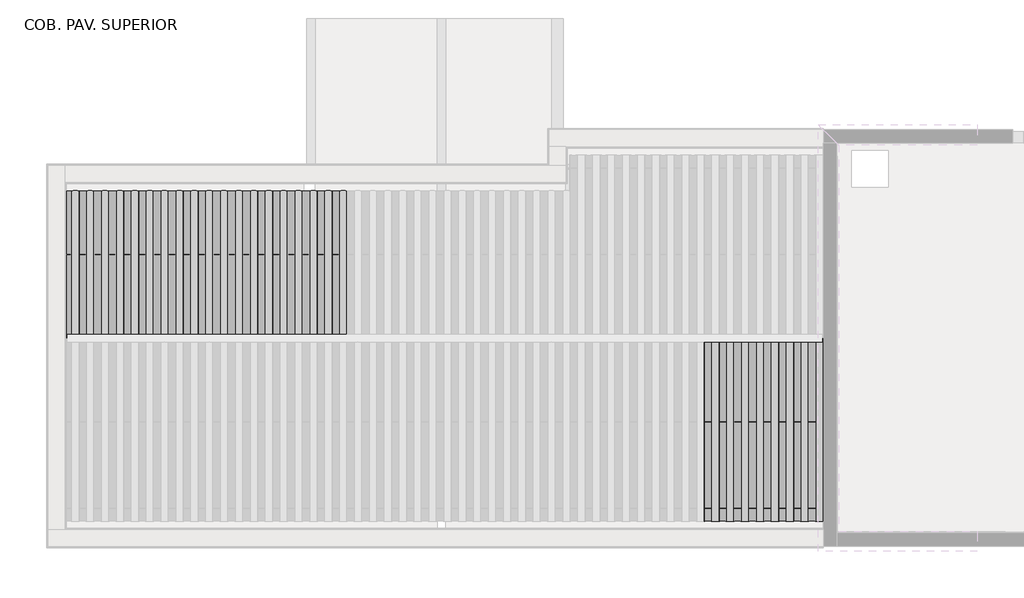
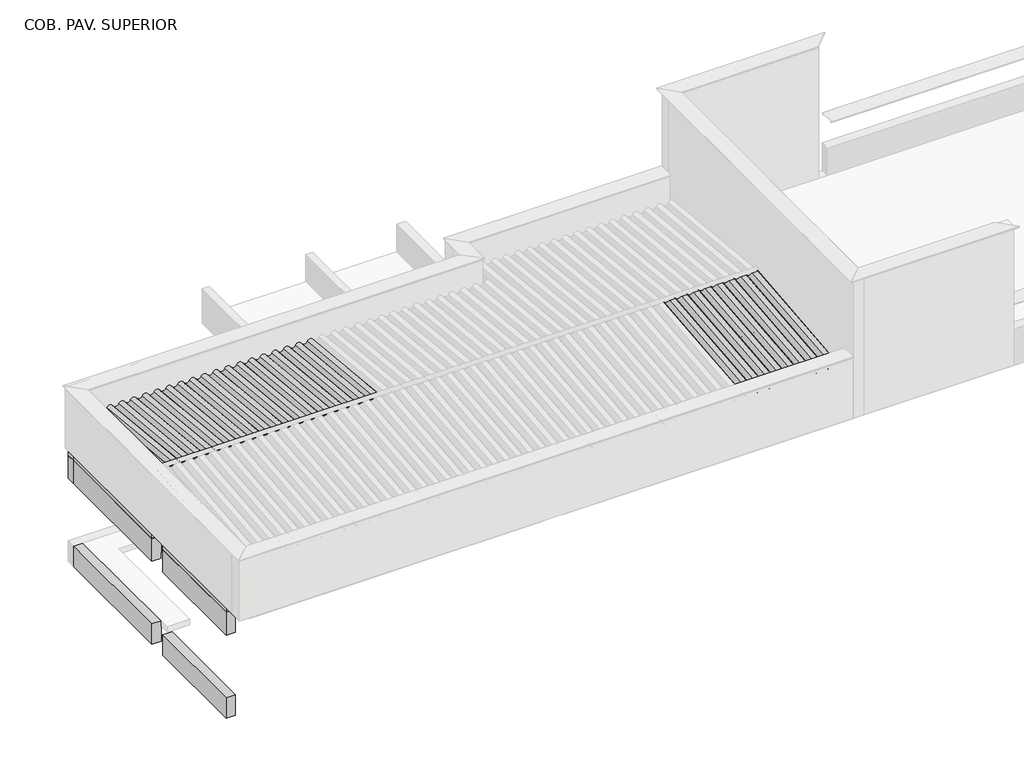
# One storey, part 3 of 7: 39 beams, 5 columns.
"""IFC4 building model written with IfcOpenShell, lengths in millimetres."""

import ifcopenshell
import ifcopenshell.guid

model = None  # the IFC model being written
_history = None  # IfcOwnerHistory: only IFC2X3 demands one
_inside = {}  # id of a spatial element -> (the spatial element, [elements in it])
_under = {}  # id of a project, library or spatial element -> (it, [spatial elements below it])
_declared = {}  # id of a project -> (the project, [libraries it declares])
_typed = {}  # id of a type object -> (the type object, [elements of that type])
_made_of = {}  # id of a material, layer set ... -> (it, [elements and type objects made of it])


def new_model(schema):
    """Start an empty IFC model of exactly this schema.

    Asked for "IFC4X3", IfcOpenShell would pick the latest addendum, in which some entities
    have other attributes; the version numbers below select the first issue.
    IFC2X3 requires an IfcOwnerHistory on every rooted entity: one is made here for all.
    """
    global model, _history
    if schema == "IFC4X3":
        model = ifcopenshell.file(schema_version=(4, 3, 0, 0))
    else:
        model = ifcopenshell.file(schema=schema)
    _inside.clear()
    _under.clear()
    _declared.clear()
    _typed.clear()
    _made_of.clear()
    _history = None
    if model.schema == "IFC2X3":
        org = make("IfcOrganization", Name="unknown")
        user = make(
            "IfcPersonAndOrganization",
            ThePerson=make("IfcPerson", FamilyName="unknown"),
            TheOrganization=org,
        )
        app = make(
            "IfcApplication",
            ApplicationDeveloper=org,
            Version="unknown",
            ApplicationFullName="unknown",
            ApplicationIdentifier="unknown",
        )
        _history = make(
            "IfcOwnerHistory",
            OwningUser=user,
            OwningApplication=app,
            ChangeAction="ADDED",
            CreationDate=0,
        )
    return model


def make(cls, **values):
    """One entity of the class cls with the attributes given. An attribute that is None is left unset."""
    return model.create_entity(
        cls, **{name: value for name, value in values.items() if value is not None}
    )


def rooted(cls, **values):
    """An entity with a GlobalId (a new one), such as an element, a storey or a relation."""
    return make(cls, GlobalId=ifcopenshell.guid.new(), OwnerHistory=_history, **values)


def si_unit(unit_type, name, prefix=None):
    """IfcSIUnit, for example si_unit("LENGTHUNIT", "METRE", prefix="MILLI")."""
    return make("IfcSIUnit", UnitType=unit_type, Prefix=prefix, Name=name)


def assignment(units):
    """IfcUnitAssignment: the units of a project."""
    return None if units is None else make("IfcUnitAssignment", Units=units)


def point(xyz):
    """IfcCartesianPoint."""
    return None if xyz is None else make("IfcCartesianPoint", Coordinates=xyz)


def direction(xyz):
    """IfcDirection."""
    return None if xyz is None else make("IfcDirection", DirectionRatios=xyz)


def frame(location, z_axis=None, x_axis=None):
    """IfcAxis2Placement3D, a coordinate frame: its origin and axes. An axis left out is left unset."""
    return make(
        "IfcAxis2Placement3D",
        Location=point(location),
        Axis=direction(z_axis),
        RefDirection=direction(x_axis),
    )


def frame_2d(location, x_axis=None):
    """IfcAxis2Placement2D, a coordinate frame in the plane: its origin and x axis."""
    return make(
        "IfcAxis2Placement2D", Location=point(location), RefDirection=direction(x_axis)
    )


def origin():
    """The frame at (0, 0, 0) with its axes left unset."""
    return frame((0.0, 0.0, 0.0))


def place(relative_to, where):
    """IfcLocalPlacement: puts the frame where relative to a parent placement (None: the world)."""
    return make(
        "IfcLocalPlacement", PlacementRelTo=relative_to, RelativePlacement=where
    )


def context(
    kind, dimensions, precision=None, world=None, true_north=None, identifier=None
):
    """IfcGeometricRepresentationContext, for example the 3D "Model" context."""
    return make(
        "IfcGeometricRepresentationContext",
        ContextIdentifier=identifier,
        ContextType=kind,
        CoordinateSpaceDimension=dimensions,
        Precision=precision,
        WorldCoordinateSystem=world,
        TrueNorth=true_north,
    )


def project(units=None, contexts=None):
    """IfcProject with its units and contexts."""
    return rooted(
        "IfcProject",
        Name="project",
        RepresentationContexts=contexts,
        UnitsInContext=assignment(units),
    )


def spatial(cls, under=None, at=None, **own):
    """A site, building, storey or space (cls), placed at a placement, below another one or the project."""
    s = rooted(cls, ObjectPlacement=at, **own)
    if under is not None:
        _under.setdefault(under.id(), (under, []))[1].append(s)
    return s


def polyline(points):
    """IfcPolyline through the points."""
    return make("IfcPolyline", Points=[point(p) for p in points])


def circle_curve(where, radius):
    """IfcCircle in the frame where."""
    return make("IfcCircle", Position=where, Radius=radius)


def trimmed(basis, trim1, trim2, sense, master):
    """IfcTrimmedCurve: the piece of a basis curve between two trims."""
    return make(
        "IfcTrimmedCurve",
        BasisCurve=basis,
        Trim1=trim1,
        Trim2=trim2,
        SenseAgreement=sense,
        MasterRepresentation=master,
    )


def segment(curve, same_sense, transition):
    """IfcCompositeCurveSegment."""
    return make(
        "IfcCompositeCurveSegment",
        Transition=transition,
        SameSense=same_sense,
        ParentCurve=curve,
    )


def composite_curve(segments, self_intersect=None):
    """IfcCompositeCurve: segments joined end to end."""
    return make("IfcCompositeCurve", Segments=segments, SelfIntersect=self_intersect)


def outline(outer, holes=None, kind="AREA"):
    """IfcArbitraryClosedProfileDef: a profile drawn as a closed curve; with holes, ...WithVoids."""
    if holes is None:
        return make("IfcArbitraryClosedProfileDef", ProfileType=kind, OuterCurve=outer)
    return make(
        "IfcArbitraryProfileDefWithVoids",
        ProfileType=kind,
        OuterCurve=outer,
        InnerCurves=holes,
    )


def extrude(swept, where, along, depth):
    """IfcExtrudedAreaSolid: the profile swept, set in the frame where, extruded along a direction by depth."""
    return make(
        "IfcExtrudedAreaSolid",
        SweptArea=swept,
        Position=where,
        ExtrudedDirection=direction(along),
        Depth=depth,
    )


def faces_of(points, faces, orient=None, outer=None):
    """IfcFace entities. A face is a list of loops; a loop is a list of indices into points, from 0.

    orient and outer hold one flag for each loop. By default every Orientation is true, the
    first loop of a face is its IfcFaceOuterBound and the others are IfcFaceBound.
    """
    made = []
    for i, loops in enumerate(faces):
        bounds = []
        for j, loop in enumerate(loops):
            is_outer = j == 0 if outer is None else outer[i][j]
            bounds.append(
                make(
                    "IfcFaceOuterBound" if is_outer else "IfcFaceBound",
                    Bound=make("IfcPolyLoop", Polygon=[points[k] for k in loop]),
                    Orientation=True if orient is None else orient[i][j],
                )
            )
        made.append(make("IfcFace", Bounds=bounds))
    return made


def faceted_brep(points, faces, orient=None, outer=None, voids=None):
    """IfcFacetedBrep: a solid bounded by flat faces; with voids (closed shells), ...WithVoids."""
    shared = [point(p) for p in points]
    hull = make("IfcClosedShell", CfsFaces=faces_of(shared, faces, orient, outer))
    if voids is None:
        return make("IfcFacetedBrep", Outer=hull)
    return make(
        "IfcFacetedBrepWithVoids",
        Outer=hull,
        Voids=[
            make(cls, CfsFaces=faces_of(shared, fs, o, b)) for cls, fs, o, b in voids
        ],
    )


def shape(context_of_items, identifier, shape_type, items):
    """IfcShapeRepresentation: the items that make up one representation, for example the "Body"."""
    return make(
        "IfcShapeRepresentation",
        ContextOfItems=context_of_items,
        RepresentationIdentifier=identifier,
        RepresentationType=shape_type,
        Items=items,
    )


def source(mapping_origin, context_of_items, identifier, shape_type, items):
    """IfcRepresentationMap: a shape defined once, which mapped items show again and again."""
    return make(
        "IfcRepresentationMap",
        MappingOrigin=mapping_origin,
        MappedRepresentation=shape(context_of_items, identifier, shape_type, items),
    )


def transform(
    local_origin,
    x_axis=None,
    y_axis=None,
    z_axis=None,
    scale=None,
    scale2=None,
    scale3=None,
    uniform=True,
):
    """IfcCartesianTransformationOperator3D, or its non-uniform kind. x_axis, y_axis, z_axis: its Axis1, 2, 3."""
    if uniform:
        return make(
            "IfcCartesianTransformationOperator3D",
            Axis1=direction(x_axis),
            Axis2=direction(y_axis),
            LocalOrigin=point(local_origin),
            Scale=scale,
            Axis3=direction(z_axis),
        )
    return make(
        "IfcCartesianTransformationOperator3DnonUniform",
        Axis1=direction(x_axis),
        Axis2=direction(y_axis),
        LocalOrigin=point(local_origin),
        Scale=scale,
        Axis3=direction(z_axis),
        Scale2=scale2,
        Scale3=scale3,
    )


def mapped(mapping_source, mapping_target):
    """IfcMappedItem: shows the shape of a source again, moved by a transform."""
    return make(
        "IfcMappedItem", MappingSource=mapping_source, MappingTarget=mapping_target
    )


def made_of(thing, what):
    """Note that an element or type object is made of a material, layer set ...; save() writes the relation."""
    if what is not None:
        _made_of.setdefault(what.id(), (what, []))[1].append(thing)
    return thing


def element(
    cls,
    number,
    at=None,
    inside=None,
    cuts=None,
    type_object=None,
    material=None,
    context=None,
    identifier="Body",
    shape_type=None,
    held_by="IfcProductDefinitionShape",
    body=None,
    shapes=None,
    **own,
):
    """One element of the class cls, such as IfcWall. Its Tag is "e" and its number.

    at: its placement. inside: the storey or other place that contains it. cuts: it is an
    opening in that element (IfcRelVoidsElement). A single representation is given by context,
    identifier, shape_type and body (its items); several are given by shapes. held_by: the class
    of the entity that holds the representations. save() writes the other relations.
    """
    e = rooted(cls, Tag="e%d" % number, ObjectPlacement=at, **own)
    if body is not None:
        shapes = [shape(context, identifier, shape_type, body)]
    if shapes is not None:
        e.Representation = make(held_by, Representations=shapes)
    if inside is not None:
        _inside.setdefault(inside.id(), (inside, []))[1].append(e)
    if cuts is not None:
        rooted(
            "IfcRelVoidsElement", RelatingBuildingElement=cuts, RelatedOpeningElement=e
        )
    if type_object is not None:
        _typed.setdefault(type_object.id(), (type_object, []))[1].append(e)
    return made_of(e, material)


def aggregate(whole, parts):
    """IfcRelAggregates: a whole, such as a stair, and the parts it consists of."""
    return rooted("IfcRelAggregates", RelatingObject=whole, RelatedObjects=parts)


def save(model, path):
    """Write the relations noted so far, then the file.

    IfcRelAggregates (storeys below a building ...), IfcRelContainedInSpatialStructure (elements
    in a storey), IfcRelDefinesByType, IfcRelAssociatesMaterial and IfcRelDeclares: one each for
    every whole, place, type object, material and project.
    """
    for whole, parts in _under.values():
        aggregate(whole, parts)
    for where, things in _inside.values():
        rooted(
            "IfcRelContainedInSpatialStructure",
            RelatedElements=things,
            RelatingStructure=where,
        )
    for kind, things in _typed.values():
        rooted("IfcRelDefinesByType", RelatedObjects=things, RelatingType=kind)
    for what, things in _made_of.values():
        rooted("IfcRelAssociatesMaterial", RelatedObjects=things, RelatingMaterial=what)
    for by, libraries in _declared.values():
        rooted("IfcRelDeclares", RelatingContext=by, RelatedDefinitions=libraries)
    model.write(path)


def column_d505325c(model_context):
    return source(origin(), model_context, "Body", "SweptSolid", [
        extrude(outline(polyline([(30.0, 80.0), (30.0, -80.0), (-30.0, -80.0), (-30.0, 80.0), (30.0, 80.0)])), frame((0.0, 0.0, 6710.0), z_axis=(0.0, 0.0, 1.0), x_axis=(1.0, 0.0, 0.0)), (0.0, 0.0, 1.0), 750.0),
    ])


def column_df674f92(model_context):
    return source(origin(), model_context, "Body", "SweptSolid", [
        extrude(outline(polyline([(30.0, 80.0), (30.0, -80.0), (-30.0, -80.0), (-30.0, 80.0), (30.0, 80.0)])), frame((0.0, 0.0, 6710.0), z_axis=(0.0, 0.0, 1.0), x_axis=(1.0, 0.0, 0.0)), (0.0, 0.0, 1.0), 575.0),
    ])


def column_4db371bd(model_context):
    return source(origin(), model_context, "Body", "SweptSolid", [
        extrude(outline(polyline([(30.0, 80.0), (30.0, -80.0), (-30.0, -80.0), (-30.0, 80.0), (30.0, 80.0)])), frame((0.0, 0.0, 6710.0), z_axis=(0.0, 0.0, 1.0), x_axis=(1.0, 0.0, 0.0)), (0.0, 0.0, 1.0), 660.0),
    ])


model = new_model("IFC4")

# Units and contexts
model_context = context("Model", 3, world=origin())
ifc_project = project(units=[si_unit("LENGTHUNIT", "METRE", prefix="MILLI")], contexts=[model_context])

# Site, building, storey
site = spatial("IfcSite", under=ifc_project)
building = spatial("IfcBuilding", under=site)
storey = spatial("IfcBuildingStorey", under=building, Name="COB. PAV. SUPERIOR", Elevation=6650.0)

# Beams
placement = place(None, origin())
element("IfcBeam", 1, ObjectType="Madeira de lei : Berço 6x12cm", at=placement, inside=storey, context=model_context, shape_type="SweptSolid", body=[
    extrude(outline(polyline([(-10679.281307, -7711.5607799), (-10679.281307, -7831.5607799), (-12679.281307, -7831.5607799), (-12679.281307, -7711.5607799), (-10679.281307, -7711.5607799)])), frame((0.0, 0.0, 6650.0), z_axis=(0.0, 0.0, 1.0), x_axis=(1.0, 0.0, 0.0)), (0.0, 0.0, 1.0), 60.0),
])
element("IfcBeam", 2, ObjectType="Madeira de lei : Berço 6x12cm", at=placement, inside=storey, context=model_context, shape_type="SweptSolid", body=[
    extrude(outline(polyline([(-8679.281307, -7711.5607799), (-8679.281307, -7831.5607799), (-10679.281307, -7831.5607799), (-10679.281307, -7711.5607799), (-8679.281307, -7711.5607799)])), frame((0.0, 0.0, 6650.0), z_axis=(0.0, 0.0, 1.0), x_axis=(1.0, 0.0, 0.0)), (0.0, 0.0, 1.0), 60.0),
])
element("IfcBeam", 3, ObjectType="Madeira de lei : Berço 6x12cm", at=placement, inside=storey, context=model_context, shape_type="SweptSolid", body=[
    extrude(outline(polyline([(-10679.281307, -6319.8711004), (-10679.281307, -6439.8711004), (-12679.281307, -6439.8711004), (-12679.281307, -6319.8711004), (-10679.281307, -6319.8711004)])), frame((0.0, 0.0, 6650.0), z_axis=(0.0, 0.0, 1.0), x_axis=(1.0, 0.0, 0.0)), (0.0, 0.0, 1.0), 60.0),
])
element("IfcBeam", 4, ObjectType="Madeira de lei : Berço 6x12cm", at=placement, inside=storey, context=model_context, shape_type="SweptSolid", body=[
    extrude(outline(polyline([(-10679.281307, -5488.3211004), (-10679.281307, -5608.3211004), (-12679.281307, -5608.3211004), (-12679.281307, -5488.3211004), (-10679.281307, -5488.3211004)])), frame((0.0, 0.0, 6650.0), z_axis=(0.0, 0.0, 1.0), x_axis=(1.0, 0.0, 0.0)), (0.0, 0.0, 1.0), 60.0),
])
element("IfcBeam", 5, ObjectType="Madeira de lei : Berço 6x12cm", at=placement, inside=storey, context=model_context, shape_type="SweptSolid", body=[
    extrude(outline(polyline([(-8779.281307, -6319.8711004), (-8779.281307, -6439.8711004), (-10679.281307, -6439.8711004), (-10679.281307, -6319.8711004), (-8779.281307, -6319.8711004)])), frame((0.0, 0.0, 6650.0), z_axis=(0.0, 0.0, 1.0), x_axis=(1.0, 0.0, 0.0)), (0.0, 0.0, 1.0), 60.0),
])
element("IfcBeam", 6, ObjectType="Madeira de lei : Berço 6x12cm", at=placement, inside=storey, context=model_context, shape_type="SweptSolid", body=[
    extrude(outline(polyline([(-679.281307, -9101.268869), (-679.281307, -9221.268869), (-2679.281307, -9221.268869), (-2679.281307, -9101.268869), (-679.281307, -9101.268869)])), frame((0.0, 0.0, 6650.0), z_axis=(0.0, 0.0, 1.0), x_axis=(1.0, 0.0, 0.0)), (0.0, 0.0, 1.0), 60.0),
])
element("IfcBeam", 7, ObjectType="Madeira de lei : Berço 6x12cm", at=placement, inside=storey, context=model_context, shape_type="SweptSolid", body=[
    extrude(outline(polyline([(-259.281307, -9101.268869), (-259.281307, -9221.268869), (-679.281307, -9221.268869), (-679.281307, -9101.268869), (-259.281307, -9101.268869)])), frame((0.0, 0.0, 6650.0), z_axis=(0.0, 0.0, 1.0), x_axis=(1.0, 0.0, 0.0)), (0.0, 0.0, 1.0), 60.0),
])
element("IfcBeam", 8, ObjectType="TQS - Viga retangular : 19.0 x 45.0", at=placement, inside=storey, context=model_context, shape_type="Brep", body=[
    faceted_brep([(-12930.2813069, -7975.5699847, 4480.0), (-12740.2813069, -7975.5699847, 4480.0), (-12740.2813069, -5165.5699847, 4480.0), (-12930.2813069, -5165.5699847, 4480.0), (-12740.2813069, -7975.5699847, 4030.0), (-12740.2813069, -5165.5699847, 4030.0), (-12740.2813069, -5165.5699847, 4360.0), (-12930.2813069, -7975.5699847, 4030.0), (-12930.2813069, -5165.5699847, 4030.0)], [[[0, 1, 2, 3]], [[1, 4, 5, 6, 2]], [[4, 7, 8, 5]], [[7, 0, 3, 8]], [[1, 0, 7, 4]], [[3, 2, 6, 5, 8]]]),
    faceted_brep([(-12930.2813069, -8375.5699847, 4480.0), (-12740.2813069, -8375.5699847, 4480.0), (-12740.2813069, -8375.5699847, 4030.0), (-12930.2813069, -8375.5699847, 4030.0), (-12930.2813069, -10643.5699847, 4480.0), (-12740.2813069, -10643.5699847, 4480.0), (-12740.2813069, -10643.5699847, 4030.0), (-12930.2813069, -10643.5699847, 4030.0)], [[[0, 1, 2, 3]], [[1, 0, 4, 5]], [[2, 1, 5, 6]], [[3, 2, 6, 7]], [[0, 3, 7, 4]], [[5, 4, 7, 6]]]),
])
element("IfcBeam", 9, ObjectType="TQS - Viga retangular : 19.0 x 50.0", at=placement, inside=storey, context=model_context, shape_type="Brep", body=[
    faceted_brep([(-8779.281307, -5165.5699847, 6350.0), (-8779.281307, -4975.5699847, 6350.0), (-12930.2813069, -4975.5699847, 6350.0), (-12930.2813069, -5165.5699847, 6350.0), (-12740.2813069, -5165.5699847, 6350.0), (-8779.281307, -5165.5699847, 5850.0), (-12930.2813069, -5165.5699847, 5850.0), (-12740.2813069, -5165.5699847, 5850.0), (-9711.481307, -5165.5699847, 5850.0), (-8779.281307, -4975.5699847, 5850.0), (-12930.2813069, -4975.5699847, 5850.0)], [[[0, 1, 2, 3, 4]], [[5, 0, 4, 3, 6, 7, 8]], [[9, 5, 8, 7, 6, 10]], [[1, 9, 10, 2]], [[1, 0, 5, 9]], [[3, 2, 10, 6]]]),
])
element("IfcBeam", 10, ObjectType="TQS - Viga retangular : 19.0 x 50.0", at=placement, inside=storey, context=model_context, shape_type="Brep", body=[
    faceted_brep([(-12930.2813069, -7975.5699847, 6350.0), (-12740.2813069, -7975.5699847, 6350.0), (-12740.2813069, -5165.5699847, 6350.0), (-12930.2813069, -5165.5699847, 6350.0), (-12740.2813069, -7975.5699847, 5850.0), (-12740.2813069, -5165.5699847, 5850.0), (-12740.2813069, -5165.5699847, 5970.0), (-12930.2813069, -7975.5699847, 5850.0), (-12930.2813069, -5165.5699847, 5850.0)], [[[0, 1, 2, 3]], [[1, 4, 5, 6, 2]], [[4, 7, 8, 5]], [[7, 0, 3, 8]], [[1, 0, 7, 4]], [[3, 2, 6, 5, 8]]]),
    faceted_brep([(-12930.2813069, -8375.5699847, 6350.0), (-12740.2813069, -8375.5699847, 6350.0), (-12740.2813069, -8375.5699847, 5850.0), (-12930.2813069, -8375.5699847, 5850.0), (-12930.2813069, -10643.5699847, 6350.0), (-12740.2813069, -10643.5699847, 6350.0), (-12740.2813069, -10643.5699847, 5850.0), (-12930.2813069, -10643.5699847, 5850.0)], [[[0, 1, 2, 3]], [[1, 0, 4, 5]], [[2, 1, 5, 6]], [[3, 2, 6, 7]], [[0, 3, 7, 4]], [[5, 4, 7, 6]]]),
])
element("IfcBeam", 11, ObjectType="TQS - Viga retangular : 19.0 x 90.0", at=placement, inside=storey, context=model_context, shape_type="Brep", body=[
    faceted_brep([(-8779.281307, -5165.5699847, 7260.5), (-8779.281307, -4975.5699847, 7260.5), (-12930.2813069, -4975.5699847, 7260.5), (-12930.2813069, -5165.5699847, 7260.5), (-12740.2813069, -5165.5699847, 7260.5), (-8779.281307, -5165.5699847, 6360.5), (-8779.281307, -5165.5699847, 6490.0), (-8779.281307, -5165.5699847, 6650.0), (-12930.2813069, -5165.5699847, 6360.5), (-12740.2813069, -5165.5699847, 6360.5), (-8779.281307, -4975.5699847, 6360.5), (-12930.2813069, -4975.5699847, 6360.5)], [[[0, 1, 2, 3, 4]], [[5, 6, 7, 0, 4, 3, 8, 9]], [[10, 5, 9, 8, 11]], [[1, 10, 11, 2]], [[1, 0, 7, 6, 5, 10]], [[3, 2, 11, 8]]]),
])
element("IfcBeam", 12, ObjectType="TQS - Viga retangular : 19.0 x 90.0", at=placement, inside=storey, context=model_context, shape_type="Brep", body=[
    faceted_brep([(-12930.2813069, -7975.5699847, 7260.5), (-12740.2813069, -7975.5699847, 7260.5), (-12740.2813069, -5165.5699847, 7260.5), (-12930.2813069, -5165.5699847, 7260.5), (-12740.2813069, -7975.5699847, 6360.5), (-12740.2813069, -5165.5699847, 6360.5), (-12740.2813069, -5165.5699847, 6490.0), (-12740.2813069, -5165.5699847, 6650.0), (-12930.2813069, -7975.5699847, 6360.5), (-12930.2813069, -5165.5699847, 6360.5)], [[[0, 1, 2, 3]], [[1, 4, 5, 6, 7, 2]], [[4, 8, 9, 5]], [[8, 0, 3, 9]], [[1, 0, 8, 4]], [[3, 2, 7, 6, 5, 9]]]),
    faceted_brep([(-12930.2813069, -8375.5699847, 7260.5), (-12740.2813069, -8375.5699847, 7260.5), (-12740.2813069, -8375.5699847, 6360.5), (-12930.2813069, -8375.5699847, 6360.5), (-12930.2813069, -10643.5699847, 7260.5), (-12740.2813069, -10643.5699847, 7260.5), (-12740.2813069, -10643.5699847, 6360.5), (-12930.2813069, -10643.5699847, 6360.5)], [[[0, 1, 2, 3]], [[1, 0, 4, 5]], [[2, 1, 5, 6]], [[3, 2, 6, 7]], [[0, 3, 7, 4]], [[4, 7, 6, 5]]]),
])
element("IfcBeam", 13, ObjectType="Telha Ondulada : Fibrocimento", at=placement, inside=storey, context=model_context, shape_type="SweptSolid", body=[
    extrude(outline(composite_curve([segment(trimmed(circle_curve(frame_2d((0.0, 66.7939461)), 66.7939461), [point((29.3501489, 6.7939461))], [point((29.3501489, 126.7939461))], True, "CARTESIAN"), True, "CONTINUOUS"), segment(polyline([(29.3501489, 126.7939461), (31.5472154, 131.2853711)]), True, "CONTINUOUS"), segment(trimmed(circle_curve(frame_2d((0.0, 66.7939461)), 71.7939461), [point((31.5472154, 131.2853711))], [point((31.5472154, 2.3025211))], False, "CARTESIAN"), True, "CONTINUOUS"), segment(trimmed(circle_curve(frame_2d((58.7002978, -53.2060539)), 61.7939461), [point((31.5472154, 2.3025211))], [point((31.5472154, -108.7146289))], True, "CARTESIAN"), True, "CONTINUOUS"), segment(polyline([(31.5472154, -108.7146289), (29.3501489, -113.2060539)]), True, "CONTINUOUS"), segment(trimmed(circle_curve(frame_2d((58.7002978, -53.2060539)), 66.7939461), [point((29.3501489, -113.2060539))], [point((29.3501489, 6.7939461))], False, "CARTESIAN"), True, "CONTINUOUS")], self_intersect=False)), frame((-2071.8843743, -10781.9594023, 7394.5315886), z_axis=(0.0, 0.9950371902099894, 0.09950371902099743), x_axis=(0.0, 0.09950371902099743, -0.9950371902099894)), (0.0, 0.0, 1.0), 3017.2295147),
])
element("IfcBeam", 14, ObjectType="Telha Ondulada : Fibrocimento", at=placement, inside=storey, context=model_context, shape_type="SweptSolid", body=[
    extrude(outline(composite_curve([segment(trimmed(circle_curve(frame_2d((0.0, 66.7939461)), 66.7939461), [point((29.3501489, 6.7939461))], [point((29.3501489, 126.7939461))], True, "CARTESIAN"), True, "CONTINUOUS"), segment(polyline([(29.3501489, 126.7939461), (31.5472154, 131.2853711)]), True, "CONTINUOUS"), segment(trimmed(circle_curve(frame_2d((0.0, 66.7939461)), 71.7939461), [point((31.5472154, 131.2853711))], [point((31.5472154, 2.3025211))], False, "CARTESIAN"), True, "CONTINUOUS"), segment(trimmed(circle_curve(frame_2d((58.7002978, -53.2060539)), 61.7939461), [point((31.5472154, 2.3025211))], [point((31.5472154, -108.7146289))], True, "CARTESIAN"), True, "CONTINUOUS"), segment(polyline([(31.5472154, -108.7146289), (29.3501489, -113.2060539)]), True, "CONTINUOUS"), segment(trimmed(circle_curve(frame_2d((58.7002978, -53.2060539)), 66.7939461), [point((29.3501489, -113.2060539))], [point((29.3501489, 6.7939461))], False, "CARTESIAN"), True, "CONTINUOUS")], self_intersect=False)), frame((-1827.3843743, -10781.9594023, 7394.5315886), z_axis=(0.0, 0.9950371902099894, 0.09950371902099743), x_axis=(0.0, 0.09950371902099743, -0.9950371902099894)), (0.0, 0.0, 1.0), 3017.2295147),
])
element("IfcBeam", 15, ObjectType="Telha Ondulada : Fibrocimento", at=placement, inside=storey, context=model_context, shape_type="SweptSolid", body=[
    extrude(outline(composite_curve([segment(trimmed(circle_curve(frame_2d((0.0, 66.7939461)), 66.7939461), [point((29.3501489, 6.7939461))], [point((29.3501489, 126.7939461))], True, "CARTESIAN"), True, "CONTINUOUS"), segment(polyline([(29.3501489, 126.7939461), (31.5472154, 131.2853711)]), True, "CONTINUOUS"), segment(trimmed(circle_curve(frame_2d((0.0, 66.7939461)), 71.7939461), [point((31.5472154, 131.2853711))], [point((31.5472154, 2.3025211))], False, "CARTESIAN"), True, "CONTINUOUS"), segment(trimmed(circle_curve(frame_2d((58.7002978, -53.2060539)), 61.7939461), [point((31.5472154, 2.3025211))], [point((31.5472154, -108.7146289))], True, "CARTESIAN"), True, "CONTINUOUS"), segment(polyline([(31.5472154, -108.7146289), (29.3501489, -113.2060539)]), True, "CONTINUOUS"), segment(trimmed(circle_curve(frame_2d((58.7002978, -53.2060539)), 66.7939461), [point((29.3501489, -113.2060539))], [point((29.3501489, 6.7939461))], False, "CARTESIAN"), True, "CONTINUOUS")], self_intersect=False)), frame((-1582.8843743, -10781.9594023, 7394.5315886), z_axis=(0.0, 0.9950371902099894, 0.0995037190209974), x_axis=(0.0, 0.0995037190209974, -0.9950371902099894)), (0.0, 0.0, 1.0), 3017.2295147),
])
element("IfcBeam", 16, ObjectType="Telha Ondulada : Fibrocimento", at=placement, inside=storey, context=model_context, shape_type="SweptSolid", body=[
    extrude(outline(composite_curve([segment(trimmed(circle_curve(frame_2d((0.0, 66.7939461)), 66.7939461), [point((29.3501489, 6.7939461))], [point((29.3501489, 126.7939461))], True, "CARTESIAN"), True, "CONTINUOUS"), segment(polyline([(29.3501489, 126.7939461), (31.5472154, 131.2853711)]), True, "CONTINUOUS"), segment(trimmed(circle_curve(frame_2d((0.0, 66.7939461)), 71.7939461), [point((31.5472154, 131.2853711))], [point((31.5472154, 2.3025211))], False, "CARTESIAN"), True, "CONTINUOUS"), segment(trimmed(circle_curve(frame_2d((58.7002978, -53.2060539)), 61.7939461), [point((31.5472154, 2.3025211))], [point((31.5472154, -108.7146289))], True, "CARTESIAN"), True, "CONTINUOUS"), segment(polyline([(31.5472154, -108.7146289), (29.3501489, -113.2060539)]), True, "CONTINUOUS"), segment(trimmed(circle_curve(frame_2d((58.7002978, -53.2060539)), 66.7939461), [point((29.3501489, -113.2060539))], [point((29.3501489, 6.7939461))], False, "CARTESIAN"), True, "CONTINUOUS")], self_intersect=False)), frame((-1338.3843743, -10781.9594023, 7394.5315886), z_axis=(0.0, 0.9950371902099894, 0.09950371902099736), x_axis=(0.0, 0.09950371902099736, -0.9950371902099894)), (0.0, 0.0, 1.0), 3017.2295147),
])
element("IfcBeam", 17, ObjectType="Telha Ondulada : Fibrocimento", at=placement, inside=storey, context=model_context, shape_type="SweptSolid", body=[
    extrude(outline(composite_curve([segment(trimmed(circle_curve(frame_2d((0.0, 66.7939461)), 66.7939461), [point((29.3501489, 6.7939461))], [point((29.3501489, 126.7939461))], True, "CARTESIAN"), True, "CONTINUOUS"), segment(polyline([(29.3501489, 126.7939461), (31.5472154, 131.2853711)]), True, "CONTINUOUS"), segment(trimmed(circle_curve(frame_2d((0.0, 66.7939461)), 71.7939461), [point((31.5472154, 131.2853711))], [point((31.5472154, 2.3025211))], False, "CARTESIAN"), True, "CONTINUOUS"), segment(trimmed(circle_curve(frame_2d((58.7002978, -53.2060539)), 61.7939461), [point((31.5472154, 2.3025211))], [point((31.5472154, -108.7146289))], True, "CARTESIAN"), True, "CONTINUOUS"), segment(polyline([(31.5472154, -108.7146289), (29.3501489, -113.2060539)]), True, "CONTINUOUS"), segment(trimmed(circle_curve(frame_2d((58.7002978, -53.2060539)), 66.7939461), [point((29.3501489, -113.2060539))], [point((29.3501489, 6.7939461))], False, "CARTESIAN"), True, "CONTINUOUS")], self_intersect=False)), frame((-1093.8843743, -10781.9594023, 7394.5315886), z_axis=(0.0, 0.9950371902099894, 0.09950371902099743), x_axis=(0.0, 0.09950371902099743, -0.9950371902099894)), (0.0, 0.0, 1.0), 3017.2295147),
])
element("IfcBeam", 18, ObjectType="Telha Ondulada : Fibrocimento", at=placement, inside=storey, context=model_context, shape_type="SweptSolid", body=[
    extrude(outline(composite_curve([segment(trimmed(circle_curve(frame_2d((0.0, 66.7939461)), 66.7939461), [point((29.3501489, 6.7939461))], [point((29.3501489, 126.7939461))], True, "CARTESIAN"), True, "CONTINUOUS"), segment(polyline([(29.3501489, 126.7939461), (31.5472154, 131.2853711)]), True, "CONTINUOUS"), segment(trimmed(circle_curve(frame_2d((0.0, 66.7939461)), 71.7939461), [point((31.5472154, 131.2853711))], [point((31.5472154, 2.3025211))], False, "CARTESIAN"), True, "CONTINUOUS"), segment(trimmed(circle_curve(frame_2d((58.7002978, -53.2060539)), 61.7939461), [point((31.5472154, 2.3025211))], [point((31.5472154, -108.7146289))], True, "CARTESIAN"), True, "CONTINUOUS"), segment(polyline([(31.5472154, -108.7146289), (29.3501489, -113.2060539)]), True, "CONTINUOUS"), segment(trimmed(circle_curve(frame_2d((58.7002978, -53.2060539)), 66.7939461), [point((29.3501489, -113.2060539))], [point((29.3501489, 6.7939461))], False, "CARTESIAN"), True, "CONTINUOUS")], self_intersect=False)), frame((-849.3843743, -10781.9594023, 7394.5315886), z_axis=(0.0, 0.9950371902099894, 0.09950371902099743), x_axis=(0.0, 0.09950371902099743, -0.9950371902099894)), (0.0, 0.0, 1.0), 3017.2295147),
])
element("IfcBeam", 19, ObjectType="Telha Ondulada : Fibrocimento", at=placement, inside=storey, context=model_context, shape_type="SweptSolid", body=[
    extrude(outline(composite_curve([segment(trimmed(circle_curve(frame_2d((0.0, 66.7939461)), 66.7939461), [point((29.3501489, 6.7939461))], [point((29.3501489, 126.7939461))], True, "CARTESIAN"), True, "CONTINUOUS"), segment(polyline([(29.3501489, 126.7939461), (31.5472154, 131.2853711)]), True, "CONTINUOUS"), segment(trimmed(circle_curve(frame_2d((0.0, 66.7939461)), 71.7939461), [point((31.5472154, 131.2853711))], [point((31.5472154, 2.3025211))], False, "CARTESIAN"), True, "CONTINUOUS"), segment(trimmed(circle_curve(frame_2d((58.7002978, -53.2060539)), 61.7939461), [point((31.5472154, 2.3025211))], [point((31.5472154, -108.7146289))], True, "CARTESIAN"), True, "CONTINUOUS"), segment(polyline([(31.5472154, -108.7146289), (29.3501489, -113.2060539)]), True, "CONTINUOUS"), segment(trimmed(circle_curve(frame_2d((58.7002978, -53.2060539)), 66.7939461), [point((29.3501489, -113.2060539))], [point((29.3501489, 6.7939461))], False, "CARTESIAN"), True, "CONTINUOUS")], self_intersect=False)), frame((-604.8843743, -10781.9594023, 7394.5315886), z_axis=(0.0, 0.9950371902099894, 0.09950371902099743), x_axis=(0.0, 0.09950371902099743, -0.9950371902099894)), (0.0, 0.0, 1.0), 3017.2295147),
])
element("IfcBeam", 20, ObjectType="Telha Ondulada : Fibrocimento", at=placement, inside=storey, context=model_context, shape_type="SweptSolid", body=[
    extrude(outline(composite_curve([segment(trimmed(circle_curve(frame_2d((0.0, 66.7939461)), 66.7939461), [point((29.3501489, 6.7939461))], [point((29.3501489, 126.7939461))], True, "CARTESIAN"), True, "CONTINUOUS"), segment(polyline([(29.3501489, 126.7939461), (31.5472154, 131.2853711)]), True, "CONTINUOUS"), segment(trimmed(circle_curve(frame_2d((0.0, 66.7939461)), 71.7939461), [point((31.5472154, 131.2853711))], [point((31.5472154, 2.3025211))], False, "CARTESIAN"), True, "CONTINUOUS"), segment(trimmed(circle_curve(frame_2d((58.7002978, -53.2060539)), 61.7939461), [point((31.5472154, 2.3025211))], [point((31.5472154, -108.7146289))], True, "CARTESIAN"), True, "CONTINUOUS"), segment(polyline([(31.5472154, -108.7146289), (29.3501489, -113.2060539)]), True, "CONTINUOUS"), segment(trimmed(circle_curve(frame_2d((58.7002978, -53.2060539)), 66.7939461), [point((29.3501489, -113.2060539))], [point((29.3501489, 6.7939461))], False, "CARTESIAN"), True, "CONTINUOUS")], self_intersect=False)), frame((-360.3843743, -10781.9594023, 7394.5315886), z_axis=(0.0, 0.9950371902099894, 0.09950371902099743), x_axis=(0.0, 0.09950371902099743, -0.9950371902099894)), (0.0, 0.0, 1.0), 3017.2295147),
])
element("IfcBeam", 21, ObjectType="Telha Ondulada : Fibrocimento", at=placement, inside=storey, context=model_context, shape_type="SweptSolid", body=[
    extrude(outline(composite_curve([segment(trimmed(circle_curve(frame_2d((-58.7002978, -53.2060539)), 66.7939461), [point((-29.3501489, 6.7939461))], [point((-29.3501489, -113.2060539))], False, "CARTESIAN"), True, "CONTINUOUS"), segment(polyline([(-29.3501489, -113.2060539), (-31.5472154, -108.7146289)]), True, "CONTINUOUS"), segment(trimmed(circle_curve(frame_2d((-58.7002978, -53.2060539)), 61.7939461), [point((-31.5472154, -108.7146289))], [point((-31.5472154, 2.3025211))], True, "CARTESIAN"), True, "CONTINUOUS"), segment(trimmed(circle_curve(frame_2d((0.0, 66.7939461)), 71.7939461), [point((-31.5472154, 2.3025211))], [point((-31.5472154, 131.2853711))], False, "CARTESIAN"), True, "CONTINUOUS"), segment(polyline([(-31.5472154, 131.2853711), (-29.3501489, 126.7939461)]), True, "CONTINUOUS"), segment(trimmed(circle_curve(frame_2d((0.0, 66.7939461)), 66.7939461), [point((-29.3501489, 126.7939461))], [point((-29.3501489, 6.7939461))], True, "CARTESIAN"), True, "CONTINUOUS")], self_intersect=False)), frame((-12585.3843743, -5348.1805671, 7453.4315886), z_axis=(0.0, -0.9950371902099893, 0.09950371902099772), x_axis=(0.0, 0.09950371902099772, 0.9950371902099893)), (0.0, 0.0, 1.0), 2425.2918406),
])
element("IfcBeam", 22, ObjectType="Telha Ondulada : Fibrocimento", at=placement, inside=storey, context=model_context, shape_type="SweptSolid", body=[
    extrude(outline(composite_curve([segment(trimmed(circle_curve(frame_2d((-58.7002978, -53.2060539)), 66.7939461), [point((-29.3501489, 6.7939461))], [point((-29.3501489, -113.2060539))], False, "CARTESIAN"), True, "CONTINUOUS"), segment(polyline([(-29.3501489, -113.2060539), (-31.5472154, -108.7146289)]), True, "CONTINUOUS"), segment(trimmed(circle_curve(frame_2d((-58.7002978, -53.2060539)), 61.7939461), [point((-31.5472154, -108.7146289))], [point((-31.5472154, 2.3025211))], True, "CARTESIAN"), True, "CONTINUOUS"), segment(trimmed(circle_curve(frame_2d((0.0, 66.7939461)), 71.7939461), [point((-31.5472154, 2.3025211))], [point((-31.5472154, 131.2853711))], False, "CARTESIAN"), True, "CONTINUOUS"), segment(polyline([(-31.5472154, 131.2853711), (-29.3501489, 126.7939461)]), True, "CONTINUOUS"), segment(trimmed(circle_curve(frame_2d((0.0, 66.7939461)), 66.7939461), [point((-29.3501489, 126.7939461))], [point((-29.3501489, 6.7939461))], True, "CARTESIAN"), True, "CONTINUOUS")], self_intersect=False)), frame((-12340.8843743, -5348.1805671, 7453.4315886), z_axis=(0.0, -0.9950371902099893, 0.09950371902099772), x_axis=(0.0, 0.09950371902099772, 0.9950371902099893)), (0.0, 0.0, 1.0), 2425.2918406),
])
element("IfcBeam", 23, ObjectType="Telha Ondulada : Fibrocimento", at=placement, inside=storey, context=model_context, shape_type="SweptSolid", body=[
    extrude(outline(composite_curve([segment(trimmed(circle_curve(frame_2d((-58.7002978, -53.2060539)), 66.7939461), [point((-29.3501489, 6.7939461))], [point((-29.3501489, -113.2060539))], False, "CARTESIAN"), True, "CONTINUOUS"), segment(polyline([(-29.3501489, -113.2060539), (-31.5472154, -108.7146289)]), True, "CONTINUOUS"), segment(trimmed(circle_curve(frame_2d((-58.7002978, -53.2060539)), 61.7939461), [point((-31.5472154, -108.7146289))], [point((-31.5472154, 2.3025211))], True, "CARTESIAN"), True, "CONTINUOUS"), segment(trimmed(circle_curve(frame_2d((0.0, 66.7939461)), 71.7939461), [point((-31.5472154, 2.3025211))], [point((-31.5472154, 131.2853711))], False, "CARTESIAN"), True, "CONTINUOUS"), segment(polyline([(-31.5472154, 131.2853711), (-29.3501489, 126.7939461)]), True, "CONTINUOUS"), segment(trimmed(circle_curve(frame_2d((0.0, 66.7939461)), 66.7939461), [point((-29.3501489, 126.7939461))], [point((-29.3501489, 6.7939461))], True, "CARTESIAN"), True, "CONTINUOUS")], self_intersect=False)), frame((-12096.3843743, -5348.1805671, 7453.4315886), z_axis=(0.0, -0.9950371902099893, 0.09950371902099768), x_axis=(0.0, 0.09950371902099768, 0.9950371902099893)), (0.0, 0.0, 1.0), 2425.2918406),
])
element("IfcBeam", 24, ObjectType="Telha Ondulada : Fibrocimento", at=placement, inside=storey, context=model_context, shape_type="SweptSolid", body=[
    extrude(outline(composite_curve([segment(trimmed(circle_curve(frame_2d((-58.7002978, -53.2060539)), 66.7939461), [point((-29.3501489, 6.7939461))], [point((-29.3501489, -113.2060539))], False, "CARTESIAN"), True, "CONTINUOUS"), segment(polyline([(-29.3501489, -113.2060539), (-31.5472154, -108.7146289)]), True, "CONTINUOUS"), segment(trimmed(circle_curve(frame_2d((-58.7002978, -53.2060539)), 61.7939461), [point((-31.5472154, -108.7146289))], [point((-31.5472154, 2.3025211))], True, "CARTESIAN"), True, "CONTINUOUS"), segment(trimmed(circle_curve(frame_2d((0.0, 66.7939461)), 71.7939461), [point((-31.5472154, 2.3025211))], [point((-31.5472154, 131.2853711))], False, "CARTESIAN"), True, "CONTINUOUS"), segment(polyline([(-31.5472154, 131.2853711), (-29.3501489, 126.7939461)]), True, "CONTINUOUS"), segment(trimmed(circle_curve(frame_2d((0.0, 66.7939461)), 66.7939461), [point((-29.3501489, 126.7939461))], [point((-29.3501489, 6.7939461))], True, "CARTESIAN"), True, "CONTINUOUS")], self_intersect=False)), frame((-11851.8843743, -5348.1805671, 7453.4315886), z_axis=(0.0, -0.9950371902099893, 0.09950371902099772), x_axis=(0.0, 0.09950371902099772, 0.9950371902099893)), (0.0, 0.0, 1.0), 2425.2918406),
])
element("IfcBeam", 25, ObjectType="Telha Ondulada : Fibrocimento", at=placement, inside=storey, context=model_context, shape_type="SweptSolid", body=[
    extrude(outline(composite_curve([segment(trimmed(circle_curve(frame_2d((-58.7002978, -53.2060539)), 66.7939461), [point((-29.3501489, 6.7939461))], [point((-29.3501489, -113.2060539))], False, "CARTESIAN"), True, "CONTINUOUS"), segment(polyline([(-29.3501489, -113.2060539), (-31.5472154, -108.7146289)]), True, "CONTINUOUS"), segment(trimmed(circle_curve(frame_2d((-58.7002978, -53.2060539)), 61.7939461), [point((-31.5472154, -108.7146289))], [point((-31.5472154, 2.3025211))], True, "CARTESIAN"), True, "CONTINUOUS"), segment(trimmed(circle_curve(frame_2d((0.0, 66.7939461)), 71.7939461), [point((-31.5472154, 2.3025211))], [point((-31.5472154, 131.2853711))], False, "CARTESIAN"), True, "CONTINUOUS"), segment(polyline([(-31.5472154, 131.2853711), (-29.3501489, 126.7939461)]), True, "CONTINUOUS"), segment(trimmed(circle_curve(frame_2d((0.0, 66.7939461)), 66.7939461), [point((-29.3501489, 126.7939461))], [point((-29.3501489, 6.7939461))], True, "CARTESIAN"), True, "CONTINUOUS")], self_intersect=False)), frame((-11607.3843743, -5348.1805671, 7453.4315886), z_axis=(0.0, -0.9950371902099893, 0.09950371902099772), x_axis=(0.0, 0.09950371902099772, 0.9950371902099893)), (0.0, 0.0, 1.0), 2425.2918406),
])
element("IfcBeam", 26, ObjectType="Telha Ondulada : Fibrocimento", at=placement, inside=storey, context=model_context, shape_type="SweptSolid", body=[
    extrude(outline(composite_curve([segment(trimmed(circle_curve(frame_2d((-58.7002978, -53.2060539)), 66.7939461), [point((-29.3501489, 6.7939461))], [point((-29.3501489, -113.2060539))], False, "CARTESIAN"), True, "CONTINUOUS"), segment(polyline([(-29.3501489, -113.2060539), (-31.5472154, -108.7146289)]), True, "CONTINUOUS"), segment(trimmed(circle_curve(frame_2d((-58.7002978, -53.2060539)), 61.7939461), [point((-31.5472154, -108.7146289))], [point((-31.5472154, 2.3025211))], True, "CARTESIAN"), True, "CONTINUOUS"), segment(trimmed(circle_curve(frame_2d((0.0, 66.7939461)), 71.7939461), [point((-31.5472154, 2.3025211))], [point((-31.5472154, 131.2853711))], False, "CARTESIAN"), True, "CONTINUOUS"), segment(polyline([(-31.5472154, 131.2853711), (-29.3501489, 126.7939461)]), True, "CONTINUOUS"), segment(trimmed(circle_curve(frame_2d((0.0, 66.7939461)), 66.7939461), [point((-29.3501489, 126.7939461))], [point((-29.3501489, 6.7939461))], True, "CARTESIAN"), True, "CONTINUOUS")], self_intersect=False)), frame((-11362.8843743, -5348.1805671, 7453.4315886), z_axis=(0.0, -0.9950371902099893, 0.09950371902099768), x_axis=(0.0, 0.09950371902099768, 0.9950371902099893)), (0.0, 0.0, 1.0), 2425.2918406),
])
element("IfcBeam", 27, ObjectType="Telha Ondulada : Fibrocimento", at=placement, inside=storey, context=model_context, shape_type="SweptSolid", body=[
    extrude(outline(composite_curve([segment(trimmed(circle_curve(frame_2d((-58.7002978, -53.2060539)), 66.7939461), [point((-29.3501489, 6.7939461))], [point((-29.3501489, -113.2060539))], False, "CARTESIAN"), True, "CONTINUOUS"), segment(polyline([(-29.3501489, -113.2060539), (-31.5472154, -108.7146289)]), True, "CONTINUOUS"), segment(trimmed(circle_curve(frame_2d((-58.7002978, -53.2060539)), 61.7939461), [point((-31.5472154, -108.7146289))], [point((-31.5472154, 2.3025211))], True, "CARTESIAN"), True, "CONTINUOUS"), segment(trimmed(circle_curve(frame_2d((0.0, 66.7939461)), 71.7939461), [point((-31.5472154, 2.3025211))], [point((-31.5472154, 131.2853711))], False, "CARTESIAN"), True, "CONTINUOUS"), segment(polyline([(-31.5472154, 131.2853711), (-29.3501489, 126.7939461)]), True, "CONTINUOUS"), segment(trimmed(circle_curve(frame_2d((0.0, 66.7939461)), 66.7939461), [point((-29.3501489, 126.7939461))], [point((-29.3501489, 6.7939461))], True, "CARTESIAN"), True, "CONTINUOUS")], self_intersect=False)), frame((-11118.3843743, -5348.1805671, 7453.4315886), z_axis=(0.0, -0.9950371902099893, 0.09950371902099776), x_axis=(0.0, 0.09950371902099776, 0.9950371902099893)), (0.0, 0.0, 1.0), 2425.2918406),
])
element("IfcBeam", 28, ObjectType="Telha Ondulada : Fibrocimento", at=placement, inside=storey, context=model_context, shape_type="SweptSolid", body=[
    extrude(outline(composite_curve([segment(trimmed(circle_curve(frame_2d((-58.7002978, -53.2060539)), 66.7939461), [point((-29.3501489, 6.7939461))], [point((-29.3501489, -113.2060539))], False, "CARTESIAN"), True, "CONTINUOUS"), segment(polyline([(-29.3501489, -113.2060539), (-31.5472154, -108.7146289)]), True, "CONTINUOUS"), segment(trimmed(circle_curve(frame_2d((-58.7002978, -53.2060539)), 61.7939461), [point((-31.5472154, -108.7146289))], [point((-31.5472154, 2.3025211))], True, "CARTESIAN"), True, "CONTINUOUS"), segment(trimmed(circle_curve(frame_2d((0.0, 66.7939461)), 71.7939461), [point((-31.5472154, 2.3025211))], [point((-31.5472154, 131.2853711))], False, "CARTESIAN"), True, "CONTINUOUS"), segment(polyline([(-31.5472154, 131.2853711), (-29.3501489, 126.7939461)]), True, "CONTINUOUS"), segment(trimmed(circle_curve(frame_2d((0.0, 66.7939461)), 66.7939461), [point((-29.3501489, 126.7939461))], [point((-29.3501489, 6.7939461))], True, "CARTESIAN"), True, "CONTINUOUS")], self_intersect=False)), frame((-10873.8843743, -5348.1805671, 7453.4315886), z_axis=(0.0, -0.9950371902099893, 0.09950371902099772), x_axis=(0.0, 0.09950371902099772, 0.9950371902099893)), (0.0, 0.0, 1.0), 2425.2918406),
])
element("IfcBeam", 29, ObjectType="Telha Ondulada : Fibrocimento", at=placement, inside=storey, context=model_context, shape_type="SweptSolid", body=[
    extrude(outline(composite_curve([segment(trimmed(circle_curve(frame_2d((-58.7002978, -53.2060539)), 66.7939461), [point((-29.3501489, 6.7939461))], [point((-29.3501489, -113.2060539))], False, "CARTESIAN"), True, "CONTINUOUS"), segment(polyline([(-29.3501489, -113.2060539), (-31.5472154, -108.7146289)]), True, "CONTINUOUS"), segment(trimmed(circle_curve(frame_2d((-58.7002978, -53.2060539)), 61.7939461), [point((-31.5472154, -108.7146289))], [point((-31.5472154, 2.3025211))], True, "CARTESIAN"), True, "CONTINUOUS"), segment(trimmed(circle_curve(frame_2d((0.0, 66.7939461)), 71.7939461), [point((-31.5472154, 2.3025211))], [point((-31.5472154, 131.2853711))], False, "CARTESIAN"), True, "CONTINUOUS"), segment(polyline([(-31.5472154, 131.2853711), (-29.3501489, 126.7939461)]), True, "CONTINUOUS"), segment(trimmed(circle_curve(frame_2d((0.0, 66.7939461)), 66.7939461), [point((-29.3501489, 126.7939461))], [point((-29.3501489, 6.7939461))], True, "CARTESIAN"), True, "CONTINUOUS")], self_intersect=False)), frame((-10629.3843743, -5348.1805671, 7453.4315886), z_axis=(0.0, -0.9950371902099893, 0.09950371902099772), x_axis=(0.0, 0.09950371902099772, 0.9950371902099893)), (0.0, 0.0, 1.0), 2425.2918406),
])
element("IfcBeam", 30, ObjectType="Telha Ondulada : Fibrocimento", at=placement, inside=storey, context=model_context, shape_type="SweptSolid", body=[
    extrude(outline(composite_curve([segment(trimmed(circle_curve(frame_2d((-58.7002978, -53.2060539)), 66.7939461), [point((-29.3501489, 6.7939461))], [point((-29.3501489, -113.2060539))], False, "CARTESIAN"), True, "CONTINUOUS"), segment(polyline([(-29.3501489, -113.2060539), (-31.5472154, -108.7146289)]), True, "CONTINUOUS"), segment(trimmed(circle_curve(frame_2d((-58.7002978, -53.2060539)), 61.7939461), [point((-31.5472154, -108.7146289))], [point((-31.5472154, 2.3025211))], True, "CARTESIAN"), True, "CONTINUOUS"), segment(trimmed(circle_curve(frame_2d((0.0, 66.7939461)), 71.7939461), [point((-31.5472154, 2.3025211))], [point((-31.5472154, 131.2853711))], False, "CARTESIAN"), True, "CONTINUOUS"), segment(polyline([(-31.5472154, 131.2853711), (-29.3501489, 126.7939461)]), True, "CONTINUOUS"), segment(trimmed(circle_curve(frame_2d((0.0, 66.7939461)), 66.7939461), [point((-29.3501489, 126.7939461))], [point((-29.3501489, 6.7939461))], True, "CARTESIAN"), True, "CONTINUOUS")], self_intersect=False)), frame((-10384.8843743, -5348.1805671, 7453.4315886), z_axis=(0.0, -0.9950371902099893, 0.09950371902099772), x_axis=(0.0, 0.09950371902099772, 0.9950371902099893)), (0.0, 0.0, 1.0), 2425.2918406),
])
element("IfcBeam", 31, ObjectType="Telha Ondulada : Fibrocimento", at=placement, inside=storey, context=model_context, shape_type="SweptSolid", body=[
    extrude(outline(composite_curve([segment(trimmed(circle_curve(frame_2d((-58.7002978, -53.2060539)), 66.7939461), [point((-29.3501489, 6.7939461))], [point((-29.3501489, -113.2060539))], False, "CARTESIAN"), True, "CONTINUOUS"), segment(polyline([(-29.3501489, -113.2060539), (-31.5472154, -108.7146289)]), True, "CONTINUOUS"), segment(trimmed(circle_curve(frame_2d((-58.7002978, -53.2060539)), 61.7939461), [point((-31.5472154, -108.7146289))], [point((-31.5472154, 2.3025211))], True, "CARTESIAN"), True, "CONTINUOUS"), segment(trimmed(circle_curve(frame_2d((0.0, 66.7939461)), 71.7939461), [point((-31.5472154, 2.3025211))], [point((-31.5472154, 131.2853711))], False, "CARTESIAN"), True, "CONTINUOUS"), segment(polyline([(-31.5472154, 131.2853711), (-29.3501489, 126.7939461)]), True, "CONTINUOUS"), segment(trimmed(circle_curve(frame_2d((0.0, 66.7939461)), 66.7939461), [point((-29.3501489, 126.7939461))], [point((-29.3501489, 6.7939461))], True, "CARTESIAN"), True, "CONTINUOUS")], self_intersect=False)), frame((-10140.3843743, -5348.1805671, 7453.4315886), z_axis=(0.0, -0.9950371902099893, 0.09950371902099768), x_axis=(0.0, 0.09950371902099768, 0.9950371902099893)), (0.0, 0.0, 1.0), 2425.2918406),
])
element("IfcBeam", 32, ObjectType="Telha Ondulada : Fibrocimento", at=placement, inside=storey, context=model_context, shape_type="SweptSolid", body=[
    extrude(outline(composite_curve([segment(trimmed(circle_curve(frame_2d((-58.7002978, -53.2060539)), 66.7939461), [point((-29.3501489, 6.7939461))], [point((-29.3501489, -113.2060539))], False, "CARTESIAN"), True, "CONTINUOUS"), segment(polyline([(-29.3501489, -113.2060539), (-31.5472154, -108.7146289)]), True, "CONTINUOUS"), segment(trimmed(circle_curve(frame_2d((-58.7002978, -53.2060539)), 61.7939461), [point((-31.5472154, -108.7146289))], [point((-31.5472154, 2.3025211))], True, "CARTESIAN"), True, "CONTINUOUS"), segment(trimmed(circle_curve(frame_2d((0.0, 66.7939461)), 71.7939461), [point((-31.5472154, 2.3025211))], [point((-31.5472154, 131.2853711))], False, "CARTESIAN"), True, "CONTINUOUS"), segment(polyline([(-31.5472154, 131.2853711), (-29.3501489, 126.7939461)]), True, "CONTINUOUS"), segment(trimmed(circle_curve(frame_2d((0.0, 66.7939461)), 66.7939461), [point((-29.3501489, 126.7939461))], [point((-29.3501489, 6.7939461))], True, "CARTESIAN"), True, "CONTINUOUS")], self_intersect=False)), frame((-9895.8843743, -5348.1805671, 7453.4315886), z_axis=(0.0, -0.9950371902099893, 0.09950371902099772), x_axis=(0.0, 0.09950371902099772, 0.9950371902099893)), (0.0, 0.0, 1.0), 2425.2918406),
])
element("IfcBeam", 33, ObjectType="Telha Ondulada : Fibrocimento", at=placement, inside=storey, context=model_context, shape_type="SweptSolid", body=[
    extrude(outline(composite_curve([segment(trimmed(circle_curve(frame_2d((-58.7002978, -53.2060539)), 66.7939461), [point((-29.3501489, 6.7939461))], [point((-29.3501489, -113.2060539))], False, "CARTESIAN"), True, "CONTINUOUS"), segment(polyline([(-29.3501489, -113.2060539), (-31.5472154, -108.7146289)]), True, "CONTINUOUS"), segment(trimmed(circle_curve(frame_2d((-58.7002978, -53.2060539)), 61.7939461), [point((-31.5472154, -108.7146289))], [point((-31.5472154, 2.3025211))], True, "CARTESIAN"), True, "CONTINUOUS"), segment(trimmed(circle_curve(frame_2d((0.0, 66.7939461)), 71.7939461), [point((-31.5472154, 2.3025211))], [point((-31.5472154, 131.2853711))], False, "CARTESIAN"), True, "CONTINUOUS"), segment(polyline([(-31.5472154, 131.2853711), (-29.3501489, 126.7939461)]), True, "CONTINUOUS"), segment(trimmed(circle_curve(frame_2d((0.0, 66.7939461)), 66.7939461), [point((-29.3501489, 126.7939461))], [point((-29.3501489, 6.7939461))], True, "CARTESIAN"), True, "CONTINUOUS")], self_intersect=False)), frame((-9651.3843743, -5348.1805671, 7453.4315886), z_axis=(0.0, -0.9950371902099893, 0.09950371902099772), x_axis=(0.0, 0.09950371902099772, 0.9950371902099893)), (0.0, 0.0, 1.0), 2425.2918406),
])
element("IfcBeam", 34, ObjectType="Telha Ondulada : Fibrocimento", at=placement, inside=storey, context=model_context, shape_type="SweptSolid", body=[
    extrude(outline(composite_curve([segment(trimmed(circle_curve(frame_2d((-58.7002978, -53.2060539)), 66.7939461), [point((-29.3501489, 6.7939461))], [point((-29.3501489, -113.2060539))], False, "CARTESIAN"), True, "CONTINUOUS"), segment(polyline([(-29.3501489, -113.2060539), (-31.5472154, -108.7146289)]), True, "CONTINUOUS"), segment(trimmed(circle_curve(frame_2d((-58.7002978, -53.2060539)), 61.7939461), [point((-31.5472154, -108.7146289))], [point((-31.5472154, 2.3025211))], True, "CARTESIAN"), True, "CONTINUOUS"), segment(trimmed(circle_curve(frame_2d((0.0, 66.7939461)), 71.7939461), [point((-31.5472154, 2.3025211))], [point((-31.5472154, 131.2853711))], False, "CARTESIAN"), True, "CONTINUOUS"), segment(polyline([(-31.5472154, 131.2853711), (-29.3501489, 126.7939461)]), True, "CONTINUOUS"), segment(trimmed(circle_curve(frame_2d((0.0, 66.7939461)), 66.7939461), [point((-29.3501489, 126.7939461))], [point((-29.3501489, 6.7939461))], True, "CARTESIAN"), True, "CONTINUOUS")], self_intersect=False)), frame((-9406.8843743, -5348.1805671, 7453.4315886), z_axis=(0.0, -0.9950371902099893, 0.09950371902099768), x_axis=(0.0, 0.09950371902099768, 0.9950371902099893)), (0.0, 0.0, 1.0), 2425.2918406),
])
element("IfcBeam", 35, ObjectType="Telha Ondulada : Fibrocimento", at=placement, inside=storey, context=model_context, shape_type="SweptSolid", body=[
    extrude(outline(composite_curve([segment(trimmed(circle_curve(frame_2d((-58.7002978, -53.2060539)), 66.7939461), [point((-29.3501489, 6.7939461))], [point((-29.3501489, -113.2060539))], False, "CARTESIAN"), True, "CONTINUOUS"), segment(polyline([(-29.3501489, -113.2060539), (-31.5472154, -108.7146289)]), True, "CONTINUOUS"), segment(trimmed(circle_curve(frame_2d((-58.7002978, -53.2060539)), 61.7939461), [point((-31.5472154, -108.7146289))], [point((-31.5472154, 2.3025211))], True, "CARTESIAN"), True, "CONTINUOUS"), segment(trimmed(circle_curve(frame_2d((0.0, 66.7939461)), 71.7939461), [point((-31.5472154, 2.3025211))], [point((-31.5472154, 131.2853711))], False, "CARTESIAN"), True, "CONTINUOUS"), segment(polyline([(-31.5472154, 131.2853711), (-29.3501489, 126.7939461)]), True, "CONTINUOUS"), segment(trimmed(circle_curve(frame_2d((0.0, 66.7939461)), 66.7939461), [point((-29.3501489, 126.7939461))], [point((-29.3501489, 6.7939461))], True, "CARTESIAN"), True, "CONTINUOUS")], self_intersect=False)), frame((-9162.3843743, -5348.1805671, 7453.4315886), z_axis=(0.0, -0.9950371902099893, 0.09950371902099776), x_axis=(0.0, 0.09950371902099776, 0.9950371902099893)), (0.0, 0.0, 1.0), 2425.2918406),
])
element("IfcBeam", 36, ObjectType="Telha Ondulada : Fibrocimento", at=placement, inside=storey, context=model_context, shape_type="SweptSolid", body=[
    extrude(outline(composite_curve([segment(trimmed(circle_curve(frame_2d((-58.7002978, -53.2060539)), 66.7939461), [point((-29.3501489, 6.7939461))], [point((-29.3501489, -113.2060539))], False, "CARTESIAN"), True, "CONTINUOUS"), segment(polyline([(-29.3501489, -113.2060539), (-31.5472154, -108.7146289)]), True, "CONTINUOUS"), segment(trimmed(circle_curve(frame_2d((-58.7002978, -53.2060539)), 61.7939461), [point((-31.5472154, -108.7146289))], [point((-31.5472154, 2.3025211))], True, "CARTESIAN"), True, "CONTINUOUS"), segment(trimmed(circle_curve(frame_2d((0.0, 66.7939461)), 71.7939461), [point((-31.5472154, 2.3025211))], [point((-31.5472154, 131.2853711))], False, "CARTESIAN"), True, "CONTINUOUS"), segment(polyline([(-31.5472154, 131.2853711), (-29.3501489, 126.7939461)]), True, "CONTINUOUS"), segment(trimmed(circle_curve(frame_2d((0.0, 66.7939461)), 66.7939461), [point((-29.3501489, 126.7939461))], [point((-29.3501489, 6.7939461))], True, "CARTESIAN"), True, "CONTINUOUS")], self_intersect=False)), frame((-8917.8843743, -5348.1805671, 7453.4315886), z_axis=(0.0, -0.9950371902099893, 0.09950371902099772), x_axis=(0.0, 0.09950371902099772, 0.9950371902099893)), (0.0, 0.0, 1.0), 2425.2918406),
])
element("IfcBeam", 37, ObjectType="Telha Ondulada : Fibrocimento", at=placement, inside=storey, context=model_context, shape_type="SweptSolid", body=[
    extrude(outline(composite_curve([segment(trimmed(circle_curve(frame_2d((-58.7002978, -53.2060539)), 66.7939461), [point((-29.3501489, 6.7939461))], [point((-29.3501489, -113.2060539))], False, "CARTESIAN"), True, "CONTINUOUS"), segment(polyline([(-29.3501489, -113.2060539), (-31.5472154, -108.7146289)]), True, "CONTINUOUS"), segment(trimmed(circle_curve(frame_2d((-58.7002978, -53.2060539)), 61.7939461), [point((-31.5472154, -108.7146289))], [point((-31.5472154, 2.3025211))], True, "CARTESIAN"), True, "CONTINUOUS"), segment(trimmed(circle_curve(frame_2d((0.0, 66.7939461)), 71.7939461), [point((-31.5472154, 2.3025211))], [point((-31.5472154, 131.2853711))], False, "CARTESIAN"), True, "CONTINUOUS"), segment(polyline([(-31.5472154, 131.2853711), (-29.3501489, 126.7939461)]), True, "CONTINUOUS"), segment(trimmed(circle_curve(frame_2d((0.0, 66.7939461)), 66.7939461), [point((-29.3501489, 126.7939461))], [point((-29.3501489, 6.7939461))], True, "CARTESIAN"), True, "CONTINUOUS")], self_intersect=False)), frame((-8673.3843743, -5348.1805671, 7453.4315886), z_axis=(0.0, -0.9950371902099893, 0.09950371902099772), x_axis=(0.0, 0.09950371902099772, 0.9950371902099893)), (0.0, 0.0, 1.0), 2425.2918406),
])
element("IfcBeam", 38, ObjectType="Telha Ondulada : Fibrocimento", at=placement, inside=storey, context=model_context, shape_type="SweptSolid", body=[
    extrude(outline(composite_curve([segment(trimmed(circle_curve(frame_2d((-58.7002978, -53.2060539)), 66.7939461), [point((-29.3501489, 6.7939461))], [point((-29.3501489, -113.2060539))], False, "CARTESIAN"), True, "CONTINUOUS"), segment(polyline([(-29.3501489, -113.2060539), (-31.5472154, -108.7146289)]), True, "CONTINUOUS"), segment(trimmed(circle_curve(frame_2d((-58.7002978, -53.2060539)), 61.7939461), [point((-31.5472154, -108.7146289))], [point((-31.5472154, 2.3025211))], True, "CARTESIAN"), True, "CONTINUOUS"), segment(trimmed(circle_curve(frame_2d((0.0, 66.7939461)), 71.7939461), [point((-31.5472154, 2.3025211))], [point((-31.5472154, 131.2853711))], False, "CARTESIAN"), True, "CONTINUOUS"), segment(polyline([(-31.5472154, 131.2853711), (-29.3501489, 126.7939461)]), True, "CONTINUOUS"), segment(trimmed(circle_curve(frame_2d((0.0, 66.7939461)), 66.7939461), [point((-29.3501489, 126.7939461))], [point((-29.3501489, 6.7939461))], True, "CARTESIAN"), True, "CONTINUOUS")], self_intersect=False)), frame((-8428.8843743, -5348.1805671, 7453.4315886), z_axis=(0.0, -0.9950371902099893, 0.09950371902099772), x_axis=(0.0, 0.09950371902099772, 0.9950371902099893)), (0.0, 0.0, 1.0), 2425.2918406),
])
element("IfcBeam", 39, ObjectType="Telha Ondulada : Fibrocimento", at=placement, inside=storey, context=model_context, shape_type="SweptSolid", body=[
    extrude(outline(composite_curve([segment(trimmed(circle_curve(frame_2d((-58.7002978, -53.2060539)), 66.7939461), [point((-29.3501489, 6.7939461))], [point((-29.3501489, -113.2060539))], False, "CARTESIAN"), True, "CONTINUOUS"), segment(polyline([(-29.3501489, -113.2060539), (-31.5472154, -108.7146289)]), True, "CONTINUOUS"), segment(trimmed(circle_curve(frame_2d((-58.7002978, -53.2060539)), 61.7939461), [point((-31.5472154, -108.7146289))], [point((-31.5472154, 2.3025211))], True, "CARTESIAN"), True, "CONTINUOUS"), segment(trimmed(circle_curve(frame_2d((0.0, 66.7939461)), 71.7939461), [point((-31.5472154, 2.3025211))], [point((-31.5472154, 131.2853711))], False, "CARTESIAN"), True, "CONTINUOUS"), segment(polyline([(-31.5472154, 131.2853711), (-29.3501489, 126.7939461)]), True, "CONTINUOUS"), segment(trimmed(circle_curve(frame_2d((0.0, 66.7939461)), 66.7939461), [point((-29.3501489, 126.7939461))], [point((-29.3501489, 6.7939461))], True, "CARTESIAN"), True, "CONTINUOUS")], self_intersect=False)), frame((-8184.3843743, -5348.1805671, 7453.4315886), z_axis=(0.0, -0.9950371902099893, 0.09950371902099768), x_axis=(0.0, 0.09950371902099768, 0.9950371902099893)), (0.0, 0.0, 1.0), 2425.2918406),
])

# Columns
column_shape = column_d505325c(model_context)
element("IfcColumn", 40, ObjectType="Madeira de lei-Coluna : Pontalete 6X16cm", at=placement, inside=storey, context=model_context, shape_type="MappedRepresentation", body=[
    mapped(column_shape, transform((-9679.281307, -7771.5607799, 0.0), x_axis=(0.0, 1.0, 0.0), y_axis=(-1.0, 0.0, 0.0), z_axis=(0.0, 0.0, 1.0))),
])
column_2_shape = column_df674f92(model_context)
element("IfcColumn", 41, ObjectType="Madeira de lei-Coluna : Pontalete 6X16cm", at=placement, inside=storey, context=model_context, shape_type="MappedRepresentation", body=[
    mapped(column_2_shape, transform((-11679.281307, -5548.3211004, 0.0), x_axis=(0.0, 1.0, 0.0), y_axis=(-1.0, 0.0, 0.0), z_axis=(0.0, 0.0, 1.0))),
])
column_3_shape = column_4db371bd(model_context)
element("IfcColumn", 42, ObjectType="Madeira de lei-Coluna : Pontalete 6X16cm", at=placement, inside=storey, context=model_context, shape_type="MappedRepresentation", body=[
    mapped(column_3_shape, transform((-11679.281307, -6379.8711004, 0.0), x_axis=(0.0, 1.0, 0.0), y_axis=(-1.0, 0.0, 0.0), z_axis=(0.0, 0.0, 1.0))),
])
element("IfcColumn", 43, ObjectType="Madeira de lei-Coluna : Pontalete 6X16cm", at=placement, inside=storey, context=model_context, shape_type="MappedRepresentation", body=[
    mapped(column_3_shape, transform((-9679.281307, -6379.8711004, 0.0), x_axis=(0.0, 1.0, 0.0), y_axis=(-1.0, 0.0, 0.0), z_axis=(0.0, 0.0, 1.0))),
])
element("IfcColumn", 44, ObjectType="Madeira de lei-Coluna : Pontalete 6X16cm", at=placement, inside=storey, context=model_context, shape_type="MappedRepresentation", body=[
    mapped(column_3_shape, transform((-1679.281307, -9161.268869, 0.0), x_axis=(0.0, 1.0, 0.0), y_axis=(-1.0, 0.0, 0.0), z_axis=(0.0, 0.0, 1.0))),
])

save(model, "model.ifc")
